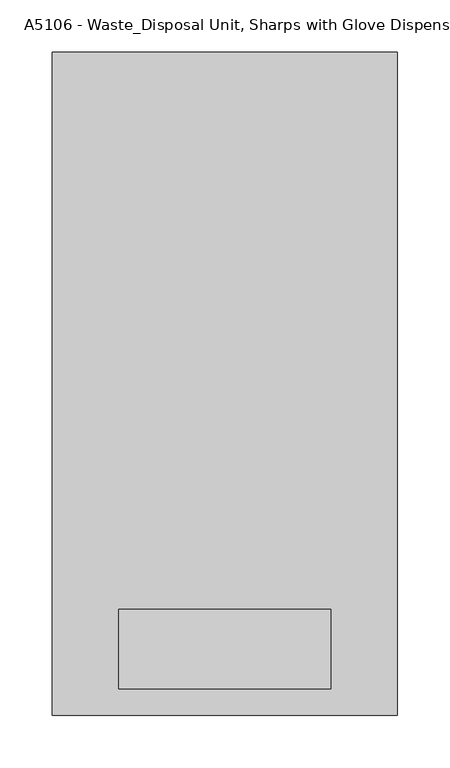
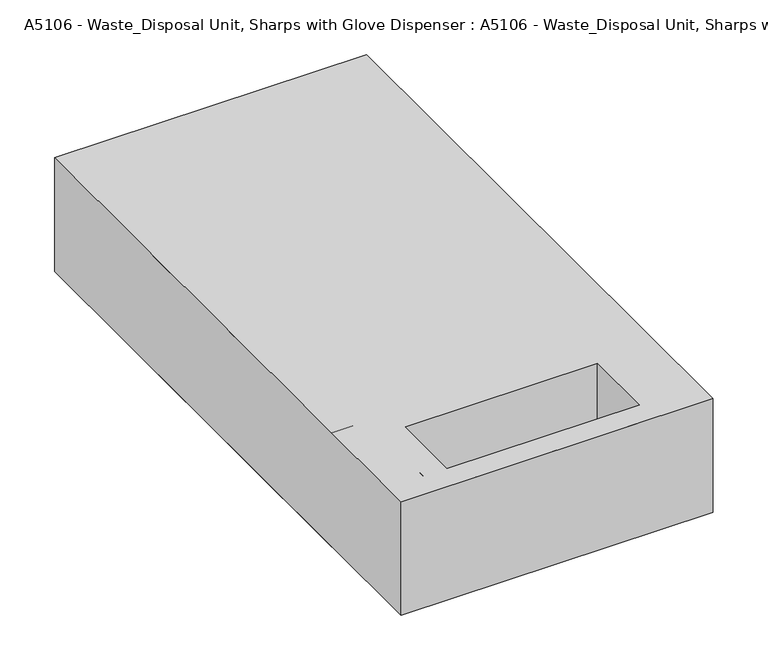
"""IFC4 building model written with IfcOpenShell, lengths in millimetres: proxy geometry, A5106 - Waste_Disposal Unit, Sharps with Glove Dispenser : A5106 - Waste_Disposal Unit, Sharps with Glove Dispenser."""

import ifcopenshell
import ifcopenshell.guid

model = None  # the IFC model being written
_history = None  # IfcOwnerHistory: only IFC2X3 demands one
_inside = {}  # id of a spatial element -> (the spatial element, [elements in it])
_under = {}  # id of a project, library or spatial element -> (it, [spatial elements below it])
_declared = {}  # id of a project -> (the project, [libraries it declares])
_typed = {}  # id of a type object -> (the type object, [elements of that type])
_made_of = {}  # id of a material, layer set ... -> (it, [elements and type objects made of it])


def new_model(schema):
    """Start an empty IFC model of exactly this schema.

    Asked for "IFC4X3", IfcOpenShell would pick the latest addendum, in which some entities
    have other attributes; the version numbers below select the first issue.
    IFC2X3 requires an IfcOwnerHistory on every rooted entity: one is made here for all.
    """
    global model, _history
    if schema == "IFC4X3":
        model = ifcopenshell.file(schema_version=(4, 3, 0, 0))
    else:
        model = ifcopenshell.file(schema=schema)
    _inside.clear()
    _under.clear()
    _declared.clear()
    _typed.clear()
    _made_of.clear()
    _history = None
    if model.schema == "IFC2X3":
        org = make("IfcOrganization", Name="unknown")
        user = make(
            "IfcPersonAndOrganization",
            ThePerson=make("IfcPerson", FamilyName="unknown"),
            TheOrganization=org,
        )
        app = make(
            "IfcApplication",
            ApplicationDeveloper=org,
            Version="unknown",
            ApplicationFullName="unknown",
            ApplicationIdentifier="unknown",
        )
        _history = make(
            "IfcOwnerHistory",
            OwningUser=user,
            OwningApplication=app,
            ChangeAction="ADDED",
            CreationDate=0,
        )
    return model


def make(cls, **values):
    """One entity of the class cls with the attributes given. An attribute that is None is left unset."""
    return model.create_entity(
        cls, **{name: value for name, value in values.items() if value is not None}
    )


def rooted(cls, **values):
    """An entity with a GlobalId (a new one), such as an element, a storey or a relation."""
    return make(cls, GlobalId=ifcopenshell.guid.new(), OwnerHistory=_history, **values)


def si_unit(unit_type, name, prefix=None):
    """IfcSIUnit, for example si_unit("LENGTHUNIT", "METRE", prefix="MILLI")."""
    return make("IfcSIUnit", UnitType=unit_type, Prefix=prefix, Name=name)


def assignment(units):
    """IfcUnitAssignment: the units of a project."""
    return None if units is None else make("IfcUnitAssignment", Units=units)


def point(xyz):
    """IfcCartesianPoint."""
    return None if xyz is None else make("IfcCartesianPoint", Coordinates=xyz)


def direction(xyz):
    """IfcDirection."""
    return None if xyz is None else make("IfcDirection", DirectionRatios=xyz)


def frame(location, z_axis=None, x_axis=None):
    """IfcAxis2Placement3D, a coordinate frame: its origin and axes. An axis left out is left unset."""
    return make(
        "IfcAxis2Placement3D",
        Location=point(location),
        Axis=direction(z_axis),
        RefDirection=direction(x_axis),
    )


def origin():
    """The frame at (0, 0, 0) with its axes left unset."""
    return frame((0.0, 0.0, 0.0))


def origin_with_axes():
    """The frame at (0, 0, 0) with the z axis (0, 0, 1) and the x axis (1, 0, 0) written out."""
    return frame((0.0, 0.0, 0.0), z_axis=(0.0, 0.0, 1.0), x_axis=(1.0, 0.0, 0.0))


def place(relative_to, where):
    """IfcLocalPlacement: puts the frame where relative to a parent placement (None: the world)."""
    return make(
        "IfcLocalPlacement", PlacementRelTo=relative_to, RelativePlacement=where
    )


def context(
    kind, dimensions, precision=None, world=None, true_north=None, identifier=None
):
    """IfcGeometricRepresentationContext, for example the 3D "Model" context."""
    return make(
        "IfcGeometricRepresentationContext",
        ContextIdentifier=identifier,
        ContextType=kind,
        CoordinateSpaceDimension=dimensions,
        Precision=precision,
        WorldCoordinateSystem=world,
        TrueNorth=true_north,
    )


def project(units=None, contexts=None):
    """IfcProject with its units and contexts."""
    return rooted(
        "IfcProject",
        Name="project",
        RepresentationContexts=contexts,
        UnitsInContext=assignment(units),
    )


def spatial(cls, under=None, at=None, **own):
    """A site, building, storey or space (cls), placed at a placement, below another one or the project."""
    s = rooted(cls, ObjectPlacement=at, **own)
    if under is not None:
        _under.setdefault(under.id(), (under, []))[1].append(s)
    return s


def polyline(points):
    """IfcPolyline through the points."""
    return make("IfcPolyline", Points=[point(p) for p in points])


def circle_curve(where, radius):
    """IfcCircle in the frame where."""
    return make("IfcCircle", Position=where, Radius=radius)


def outline(outer, holes=None, kind="AREA"):
    """IfcArbitraryClosedProfileDef: a profile drawn as a closed curve; with holes, ...WithVoids."""
    if holes is None:
        return make("IfcArbitraryClosedProfileDef", ProfileType=kind, OuterCurve=outer)
    return make(
        "IfcArbitraryProfileDefWithVoids",
        ProfileType=kind,
        OuterCurve=outer,
        InnerCurves=holes,
    )


def extrude(swept, where, along, depth):
    """IfcExtrudedAreaSolid: the profile swept, set in the frame where, extruded along a direction by depth."""
    return make(
        "IfcExtrudedAreaSolid",
        SweptArea=swept,
        Position=where,
        ExtrudedDirection=direction(along),
        Depth=depth,
    )


def shape(context_of_items, identifier, shape_type, items):
    """IfcShapeRepresentation: the items that make up one representation, for example the "Body"."""
    return make(
        "IfcShapeRepresentation",
        ContextOfItems=context_of_items,
        RepresentationIdentifier=identifier,
        RepresentationType=shape_type,
        Items=items,
    )


def source(mapping_origin, context_of_items, identifier, shape_type, items):
    """IfcRepresentationMap: a shape defined once, which mapped items show again and again."""
    return make(
        "IfcRepresentationMap",
        MappingOrigin=mapping_origin,
        MappedRepresentation=shape(context_of_items, identifier, shape_type, items),
    )


def transform(
    local_origin,
    x_axis=None,
    y_axis=None,
    z_axis=None,
    scale=None,
    scale2=None,
    scale3=None,
    uniform=True,
):
    """IfcCartesianTransformationOperator3D, or its non-uniform kind. x_axis, y_axis, z_axis: its Axis1, 2, 3."""
    if uniform:
        return make(
            "IfcCartesianTransformationOperator3D",
            Axis1=direction(x_axis),
            Axis2=direction(y_axis),
            LocalOrigin=point(local_origin),
            Scale=scale,
            Axis3=direction(z_axis),
        )
    return make(
        "IfcCartesianTransformationOperator3DnonUniform",
        Axis1=direction(x_axis),
        Axis2=direction(y_axis),
        LocalOrigin=point(local_origin),
        Scale=scale,
        Axis3=direction(z_axis),
        Scale2=scale2,
        Scale3=scale3,
    )


def mapped(mapping_source, mapping_target):
    """IfcMappedItem: shows the shape of a source again, moved by a transform."""
    return make(
        "IfcMappedItem", MappingSource=mapping_source, MappingTarget=mapping_target
    )


def made_of(thing, what):
    """Note that an element or type object is made of a material, layer set ...; save() writes the relation."""
    if what is not None:
        _made_of.setdefault(what.id(), (what, []))[1].append(thing)
    return thing


def element(
    cls,
    number,
    at=None,
    inside=None,
    cuts=None,
    type_object=None,
    material=None,
    context=None,
    identifier="Body",
    shape_type=None,
    held_by="IfcProductDefinitionShape",
    body=None,
    shapes=None,
    **own,
):
    """One element of the class cls, such as IfcWall. Its Tag is "e" and its number.

    at: its placement. inside: the storey or other place that contains it. cuts: it is an
    opening in that element (IfcRelVoidsElement). A single representation is given by context,
    identifier, shape_type and body (its items); several are given by shapes. held_by: the class
    of the entity that holds the representations. save() writes the other relations.
    """
    e = rooted(cls, Tag="e%d" % number, ObjectPlacement=at, **own)
    if body is not None:
        shapes = [shape(context, identifier, shape_type, body)]
    if shapes is not None:
        e.Representation = make(held_by, Representations=shapes)
    if inside is not None:
        _inside.setdefault(inside.id(), (inside, []))[1].append(e)
    if cuts is not None:
        rooted(
            "IfcRelVoidsElement", RelatingBuildingElement=cuts, RelatedOpeningElement=e
        )
    if type_object is not None:
        _typed.setdefault(type_object.id(), (type_object, []))[1].append(e)
    return made_of(e, material)


def aggregate(whole, parts):
    """IfcRelAggregates: a whole, such as a stair, and the parts it consists of."""
    return rooted("IfcRelAggregates", RelatingObject=whole, RelatedObjects=parts)


def save(model, path):
    """Write the relations noted so far, then the file.

    IfcRelAggregates (storeys below a building ...), IfcRelContainedInSpatialStructure (elements
    in a storey), IfcRelDefinesByType, IfcRelAssociatesMaterial and IfcRelDeclares: one each for
    every whole, place, type object, material and project.
    """
    for whole, parts in _under.values():
        aggregate(whole, parts)
    for where, things in _inside.values():
        rooted(
            "IfcRelContainedInSpatialStructure",
            RelatedElements=things,
            RelatingStructure=where,
        )
    for kind, things in _typed.values():
        rooted("IfcRelDefinesByType", RelatedObjects=things, RelatingType=kind)
    for what, things in _made_of.values():
        rooted("IfcRelAssociatesMaterial", RelatedObjects=things, RelatingMaterial=what)
    for by, libraries in _declared.values():
        rooted("IfcRelDeclares", RelatingContext=by, RelatedDefinitions=libraries)
    model.write(path)


def plane_surface(at):
    """IfcPlane: the flat surface through the origin of the frame at, square to its z axis."""
    return make("IfcPlane", Position=at)


def cylinder_surface(at, radius):
    """IfcCylindricalSurface: all points at the distance radius from the z axis of the frame at."""
    return make("IfcCylindricalSurface", Position=at, Radius=radius)


def revolved_surface(curve, axis_point, axis_direction):
    """IfcSurfaceOfRevolution: the curve turned about the line through axis_point along axis_direction."""
    return make(
        "IfcSurfaceOfRevolution",
        SweptCurve=make("IfcArbitraryOpenProfileDef", ProfileType="CURVE", Curve=curve),
        AxisPosition=make("IfcAxis1Placement", Location=point(axis_point), Axis=direction(axis_direction)),
    )


def advanced_brep(points, edges, surfaces, faces):
    """IfcAdvancedBrep: a solid bounded by faces that lie on surfaces and meet in shared edges.

    An edge is (start, end): straight between two places in points (the first is 0);
    or (start, end, curve); or (start, end, curve, False) where it runs against its curve.
    A face is (place in surfaces, loops), or (place, loops, False) where it looks against
    its surface's normal. A loop lists edges by number (the first is 1), with a minus sign
    where the edge is run from its end to its start. The first loop is the outer one.
    """
    corners = [point(p) for p in points]
    vertices = [make("IfcVertexPoint", VertexGeometry=c) for c in corners]
    made = []
    for start, end, *more in edges:
        made.append(
            make(
                "IfcEdgeCurve",
                EdgeStart=vertices[start],
                EdgeEnd=vertices[end],
                EdgeGeometry=more[0] if more else make("IfcPolyline", Points=[corners[start], corners[end]]),
                SameSense=more[1] if len(more) > 1 else True,
            )
        )
    hull = []
    for where, loops, *sense in faces:
        bounds = []
        for j, loop in enumerate(loops):
            ring = [make("IfcOrientedEdge", EdgeElement=made[abs(k) - 1], Orientation=k > 0) for k in loop]
            bounds.append(
                make(
                    "IfcFaceOuterBound" if j == 0 else "IfcFaceBound",
                    Bound=make("IfcEdgeLoop", EdgeList=ring),
                    Orientation=True,
                )
            )
        hull.append(make("IfcAdvancedFace", Bounds=bounds, FaceSurface=surfaces[where], SameSense=sense[0] if sense else True))
    return make("IfcAdvancedBrep", Outer=make("IfcClosedShell", CfsFaces=hull))


def a5106_waste_disposal_unit_sharps_with_glove_dispenser_a5106_9fb1b7a7(model_context):
    return source(origin(), model_context, "Body", "SolidModel", [
        advanced_brep(
        [(101.6, -533.4, 127.0), (101.6, -457.2, 127.0), (101.6, -457.2, 25.4), (-101.6, -457.2, 127.0), (-101.6, -533.4, 127.0), (-101.6, -457.2, 25.4), (165.1, -558.8, 127.0), (165.1, 76.2, 127.0), (-165.1, 76.2, 127.0), (-165.1, -558.8, 127.0), (165.1, -558.8, 0.0), (-165.1, -558.8, 0.0), (-165.1, 76.2, 0.0), (165.1, 76.2, 0.0)],
        [
            (0, 1),
            (1, 2),
            (2, 0, circle_curve(frame((101.6, -428.5291538, 126.2781346), z_axis=(-1.0, 0.0, 0.0), x_axis=(0.0, -1.0, 0.0)), 104.8733306)),
            (3, 4),
            (4, 5, circle_curve(frame((-101.6, -428.5291538, 126.2781346), z_axis=(1.0, 0.0, 0.0), x_axis=(0.0, -1.0, 0.0)), 104.8733306)),
            (5, 3),
            (1, 3),
            (5, 2),
            (4, 0),
            (6, 7),
            (7, 8),
            (8, 9),
            (9, 6),
            (10, 11),
            (11, 12),
            (12, 13),
            (13, 10),
            (9, 11),
            (10, 6),
            (8, 12),
            (7, 13),
        ],
        [
            plane_surface(frame((101.6, -457.2, 127.0), z_axis=(-1.0, 0.0, 0.0), x_axis=(0.0, 0.0, -1.0))),
            plane_surface(frame((-101.6, -457.2, 127.0), z_axis=(1.0, 0.0, 0.0), x_axis=(0.0, 0.0, 1.0))),
            plane_surface(frame((101.6, -457.2, 127.0), z_axis=(0.0, -1.0, 0.0), x_axis=(-1.0, 0.0, 0.0))),
            revolved_surface(polyline([(101.6, -533.4024844, 126.2781346), (-101.6, -533.4024844, 126.2781346)]), (-101.6, -428.5291538, 126.2781346), (1.0, 0.0, 0.0)),
            plane_surface(frame((-165.1, -558.8, 127.0), z_axis=(0.0, 0.0, 1.0), x_axis=(-1.0, 0.0, 0.0))),
            plane_surface(frame((-165.1, -558.8, 0.0), z_axis=(0.0, 0.0, -1.0), x_axis=(1.0, 0.0, 0.0))),
            plane_surface(frame((165.1, -558.8, 127.0), z_axis=(0.0, -1.0, 0.0), x_axis=(0.0, 0.0, -1.0))),
            plane_surface(frame((-165.1, -558.8, 127.0), z_axis=(-1.0, 0.0, 0.0), x_axis=(0.0, 0.0, -1.0))),
            plane_surface(frame((-165.1, 76.2, 127.0), z_axis=(0.0, 1.0, 0.0), x_axis=(0.0, 0.0, -1.0))),
            plane_surface(frame((165.1, 76.2, 127.0), z_axis=(1.0, 0.0, 0.0), x_axis=(0.0, 0.0, -1.0))),
        ],
        [
            (0, [[1, 2, 3]]),
            (1, [[4, 5, 6]]),
            (2, [[7, -6, 8, -2]]),
            (3, [[-8, -5, 9, -3]]),
            (4, [[10, 11, 12, 13], [-9, -4, -7, -1]]),
            (5, [[14, 15, 16, 17]]),
            (6, [[18, -14, 19, -13]]),
            (7, [[20, -15, -18, -12]]),
            (8, [[21, -16, -20, -11]]),
            (9, [[-19, -17, -21, -10]]),
        ],
    ),
        advanced_brep(
        [(127.0, -431.8, 0.0), (127.0, -431.8, 127.0), (127.0, -558.8, 127.0), (-127.0, -431.8, 0.0), (-127.0, -558.8, 127.0), (-127.0, -431.8, 127.0), (101.6, -533.4, 127.0), (-101.6, -533.4, 127.0), (-101.6, -457.2, 127.0), (101.6, -457.2, 127.0), (101.6, -457.2, 25.4), (-101.6, -457.2, 25.4)],
        [
            (0, 1),
            (1, 2),
            (2, 0, circle_curve(frame((127.0, -431.8, 127.0), z_axis=(1.0, 0.0, 0.0), x_axis=(0.0, 0.0, -1.0)), 127.0)),
            (3, 4, circle_curve(frame((-127.0, -431.8, 127.0), z_axis=(-1.0, 0.0, 0.0), x_axis=(0.0, 0.0, -1.0)), 127.0)),
            (4, 5),
            (5, 3),
            (2, 4),
            (3, 0),
            (1, 5),
            (6, 7),
            (7, 8),
            (8, 9),
            (9, 6),
            (9, 10),
            (10, 6, circle_curve(frame((101.6, -428.5291538, 126.2781346), z_axis=(-1.0, 0.0, 0.0), x_axis=(0.0, -1.0, 0.0)), 104.8733306)),
            (7, 11, circle_curve(frame((-101.6, -428.5291538, 126.2781346), z_axis=(1.0, 0.0, 0.0), x_axis=(0.0, -1.0, 0.0)), 104.8733306)),
            (11, 8),
            (11, 10),
        ],
        [
            plane_surface(frame((127.0, -431.8, 0.0), z_axis=(1.0, 0.0, 0.0), x_axis=(0.0, -1.0, 0.0))),
            plane_surface(frame((-127.0, -431.8, 0.0), z_axis=(-1.0, 0.0, 0.0), x_axis=(0.0, 1.0, 0.0))),
            cylinder_surface(frame((-127.0, -431.8, 127.0), z_axis=(1.0, 0.0, 0.0), x_axis=(0.0, 0.0, -1.0)), 127.0),
            plane_surface(frame((127.0, -558.8, 127.0), z_axis=(0.0, 0.0, 1.0), x_axis=(-1.0, 0.0, 0.0))),
            plane_surface(frame((127.0, -431.8, 127.0), z_axis=(0.0, 1.0, 0.0), x_axis=(-1.0, 0.0, 0.0))),
            plane_surface(frame((101.6, -457.2, 127.0), z_axis=(-1.0, 0.0, 0.0), x_axis=(0.0, 0.0, -1.0))),
            plane_surface(frame((-101.6, -457.2, 127.0), z_axis=(1.0, 0.0, 0.0), x_axis=(0.0, 0.0, 1.0))),
            plane_surface(frame((101.6, -457.2, 127.0), z_axis=(0.0, -1.0, 0.0), x_axis=(-1.0, 0.0, 0.0))),
            revolved_surface(polyline([(101.6, -533.4024844, 126.2781346), (-101.6, -533.4024844, 126.2781346)]), (-101.6, -428.5291538, 126.2781346), (1.0, 0.0, 0.0)),
        ],
        [
            (0, [[1, 2, 3]]),
            (1, [[4, 5, 6]]),
            (2, [[7, -4, 8, -3]]),
            (3, [[9, -5, -7, -2], [10, 11, 12, 13]]),
            (4, [[-8, -6, -9, -1]]),
            (5, [[-13, 14, 15]]),
            (6, [[-11, 16, 17]]),
            (7, [[-12, -17, 18, -14]]),
            (8, [[-18, -16, -10, -15]]),
        ],
    ),
        extrude(outline(polyline([(127.0, -76.2), (-127.0, -76.2), (-127.0, 76.2), (127.0, 76.2), (127.0, -76.2)])), origin_with_axes(), (0.0, 0.0, 1.0), 101.6),
        extrude(outline(polyline([(165.1, -431.8), (-165.1, -431.8), (-165.1, -76.2), (165.1, -76.2), (165.1, -431.8)])), origin_with_axes(), (0.0, 0.0, 1.0), 127.0),
    ])


if __name__ == "__main__":
    model = new_model("IFC4")
    model_context = context("Model", 3, world=origin())
    ifc_project = project(units=[si_unit("LENGTHUNIT", "METRE", prefix="MILLI")], contexts=[model_context])
    site = spatial("IfcSite", under=ifc_project)
    building = spatial("IfcBuilding", under=site)
    placement = place(None, origin())
    a5106_waste_disposal_unit_sharps_with_glove_dispenser_a5106_shape = a5106_waste_disposal_unit_sharps_with_glove_dispenser_a5106_9fb1b7a7(model_context)
    element("IfcBuildingElementProxy", 1, Name="A5106 - Waste_Disposal Unit, Sharps with Glove Dispenser : A5106 - Waste_Disposal Unit, Sharps with Glove Dispenser", ObjectType="A5106 - Waste_Disposal Unit, Sharps with Glove Dispenser : A5106 - Waste_Disposal Unit, Sharps with Glove Dispenser", at=placement, inside=building, context=model_context, shape_type="MappedRepresentation", body=[
        mapped(a5106_waste_disposal_unit_sharps_with_glove_dispenser_a5106_shape, transform((0.0, 0.0, 0.0), x_axis=(1.0, 0.0, 0.0), y_axis=(0.0, 1.0, 0.0), z_axis=(0.0, 0.0, 1.0))),
    ])
    save(model, "model.ifc")

# Revit data of these elements
# Type "A5106 - Waste_Disposal Unit, Sharps with Glove Dispenser : A5106 - Waste_Disposal Unit, Sharps with Glove Dispenser"
#   Watts2 = "0"
#   Watts1 = "0"
#   Unit_Issue = "EA"
#   UTIL_6_Misc = "-"
#   UTIL_5_NonMedGas = "-"
#   UTIL_4_MiscGas = "-"
#   UTIL_3_MedGas = "-"
#   UTIL_2_Elec = "-"
#   UTIL_1_WaterDrain = "-"
#   Nomenclature = "Waste Disposal Unit, Sharps w/Glove Dispenser"
#   NSN = "6530"
#   Location [instance default] = ""
#   JSN = "A5106"
#   Fund_Source_VA = "-"
#   Fund_Source_Navy = "-"
#   Fund_Source_Army = "-"
#   Fund_Source_AF = "-"
#   ELEC_Volts2 = "0"
#   ELEC_Volts1 = "0"
#   ELEC_Phase2 = "0"
#   ELEC_Phase1 = "0"
#   ELEC_HertzSwitch = "0"
#   ELEC_HertzDependent = "0"
#   ELEC_Hertz = "0"
#   ELEC_Amps2 = "0"
#   ELEC_Amps1 = "0"
#   DetailDescription = "The unit is designed for the disposal of sharps and complies with OSHA guidelines for the handling of sharps. It shall house a 5 quart container and be capable of being mounted on a wall. It shall have a glove dispenser attached. The unit shall be secured by a locked enclosure."
#   CAT_VA = "C"
#   CAT_Navy = "A"
#   CAT_IHS = "-"
#   CAT_Army = "C"
#   CAT_AF = "C"
#   BTUperhour = "0"
#   Weight_IP = 5
#   Default Elevation = 4' - 0"
#   DIM_Width_IP = 1' - 1"
#   DIM_Height_IP = 2' - 1"
#   DIM_Depth_IP = 0' - 5"
#   finish [instance default] = none
#   Assembly Code = ""
# Element 1 (IfcBuildingElementProxy, "A5106 - Waste_Disposal Unit, Sharps with Glove Dispenser : A5106 - Waste_Disposal Unit, Sharps with Glove Dispenser")
#   Location = "DNTG4"
#   Materials on its faces: "EquipSpace"
# Materials
#   "EquipSpace": class "Unassigned", colour RGB 221 217 195, transparency 0.5
